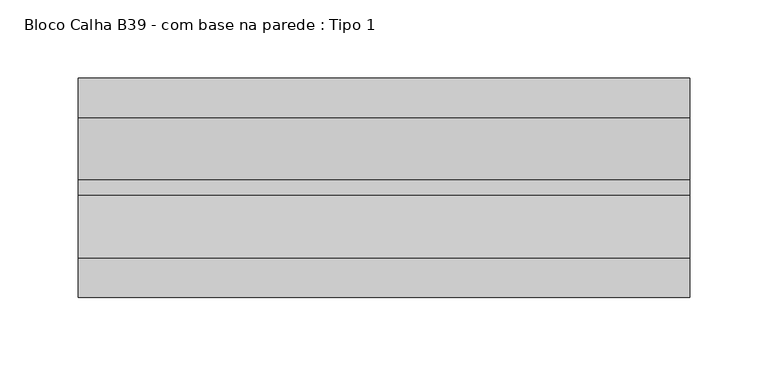
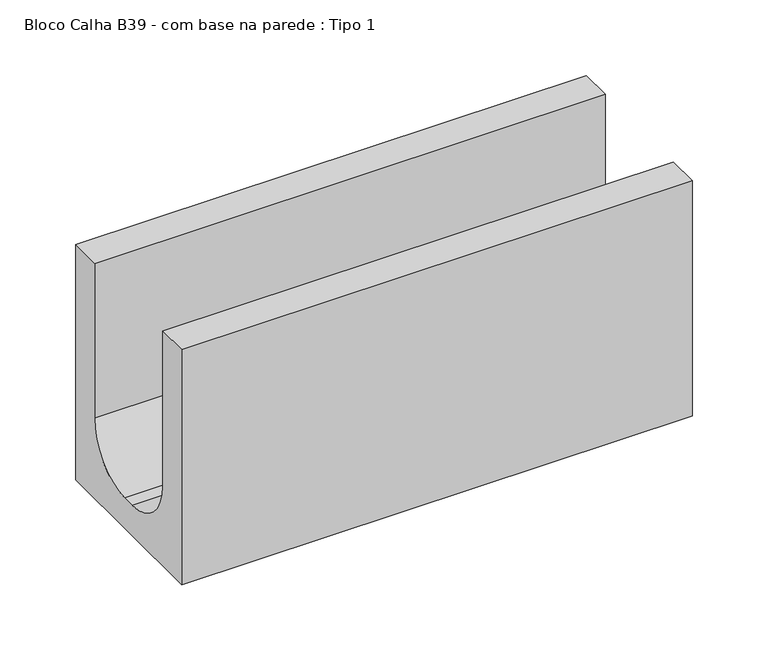
"""IFC4 building model written with IfcOpenShell, lengths in millimetres: proxy geometry, Bloco Calha B39 - com base na parede : Tipo 1."""

from ifc_helpers import new_model, si_unit, point, frame, frame_2d, origin, place, context, project, spatial, polyline, circle_curve, trimmed, segment, composite_curve, outline, extrude, source, transform, mapped, element, save


def bloco_calha_b39_com_base_na_parede_tipo_1_4603c5f3(model_context):
    return source(origin(), model_context, "Body", "SweptSolid", [
        extrude(outline(composite_curve([segment(polyline([(70.0, 0.0), (-70.0, 0.0), (-70.0, 190.0), (-45.0, 190.0), (-45.0, 65.0)]), True, "CONTINUOUS"), segment(trimmed(circle_curve(frame_2d((-5.0, 65.0)), 40.0), [point((-45.0, 65.0))], [point((-5.0, 25.0))], True, "CARTESIAN"), True, "CONTINUOUS"), segment(polyline([(-5.0, 25.0), (5.0, 25.0)]), True, "CONTINUOUS"), segment(trimmed(circle_curve(frame_2d((5.0, 65.0)), 40.0), [point((5.0, 25.0))], [point((45.0, 65.0))], True, "CARTESIAN"), True, "CONTINUOUS"), segment(polyline([(45.0, 65.0), (45.0, 190.0), (70.0, 190.0), (70.0, 0.0)]), True, "CONTINUOUS")], self_intersect=False)), frame((-70.0, 0.0, 0.0), z_axis=(1.0, 0.0, 0.0), x_axis=(0.0, 1.0, 0.0)), (0.0, 0.0, 1.0), 390.0),
    ])


if __name__ == "__main__":
    model = new_model("IFC4")
    model_context = context("Model", 3, world=origin())
    ifc_project = project(units=[si_unit("LENGTHUNIT", "METRE", prefix="MILLI")], contexts=[model_context])
    site = spatial("IfcSite", under=ifc_project)
    building = spatial("IfcBuilding", under=site)
    placement = place(None, origin())
    bloco_calha_b39_com_base_na_parede_tipo_1_shape = bloco_calha_b39_com_base_na_parede_tipo_1_4603c5f3(model_context)
    element("IfcBuildingElementProxy", 1, Name="Bloco Calha B39 - com base na parede : Tipo 1", ObjectType="Bloco Calha B39 - com base na parede : Tipo 1", at=placement, inside=building, context=model_context, shape_type="MappedRepresentation", body=[
        mapped(bloco_calha_b39_com_base_na_parede_tipo_1_shape, transform((0.0, 0.0, 0.0), x_axis=(1.0, 0.0, 0.0), y_axis=(0.0, 1.0, 0.0), z_axis=(0.0, 0.0, 1.0))),
    ])
    save(model, "model.ifc")

# Revit data of these elements
# Type "Bloco Calha B39 - com base na parede : Tipo 1"
#   SINAPI = ""
#   Assembly Code = ""
